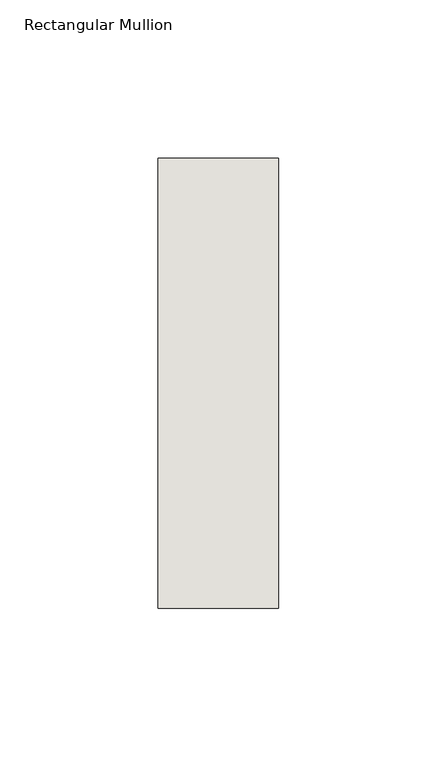
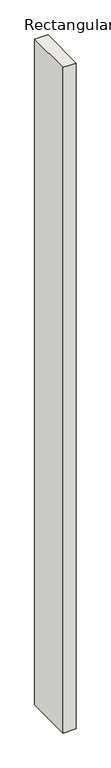
"""IFC4 building model written with IfcOpenShell, lengths in millimetres: wall geometry, Rectangular Mullion : NLRS_21_CWM_hsb-regel 38x142_gen_rsf."""

from ifc_helpers import new_model, si_unit, frame, origin, place, context, project, spatial, polyline, outline, extrude, source, transform, mapped, element, save


def rectangular_mullion_b4280be7(model_context):
    return source(origin(), model_context, "Body", "SweptSolid", [
        extrude(outline(polyline([(-38.0, -71.0), (-38.0, 71.0), (0.0, 71.0), (0.0, -71.0), (-38.0, -71.0)])), frame((0.0, 0.0, -2038.0), z_axis=(0.0, 0.0, 1.0), x_axis=(1.0, 0.0, 0.0)), (0.0, 0.0, 1.0), 2038.0),
    ])


if __name__ == "__main__":
    model = new_model("IFC4")
    model_context = context("Model", 3, world=origin())
    ifc_project = project(units=[si_unit("LENGTHUNIT", "METRE", prefix="MILLI")], contexts=[model_context])
    site = spatial("IfcSite", under=ifc_project)
    building = spatial("IfcBuilding", under=site)
    placement = place(None, origin())
    rectangular_mullion_shape = rectangular_mullion_b4280be7(model_context)
    element("IfcWall", 1, ObjectType="Rectangular Mullion : NLRS_21_CWM_hsb-regel 38x142_gen_rsf", at=placement, inside=building, context=model_context, shape_type="MappedRepresentation", body=[
        mapped(rectangular_mullion_shape, transform((0.0, 0.0, 0.0), x_axis=(1.0, 0.0, 0.0), y_axis=(0.0, 1.0, 0.0), z_axis=(0.0, 0.0, 1.0))),
    ])
    save(model, "model.ifc")

# Revit data of these elements
# Type "Rectangular Mullion : NLRS_21_CWM_hsb-regel 38x142_gen_rsf"
#   Type IfcGUID = "07M7mRoiH1CR8m_RSKIwpF"
#   Assembly Code = "21.10"
#   IfcExportAs = "IfcWall"
#   built-in parameter 1007322 = 0.465879 (stored number, unit not read)
#   built-in parameter 1007321 = 0.062336 (stored number, unit not read)
#   built-in parameter 1007320 = 0.062336 (stored number, unit not read)
# Element 1 (IfcWall, "Rectangular Mullion : NLRS_21_CWM_hsb-regel 38x142_gen_rsf")
#   Materials on its faces: "NLRS_i2_hout naaldhout vuren_gen_rsf"
# Materials
#   "NLRS_i2_hout naaldhout vuren_gen_rsf": class "I - Hout", colour RGB 234 199 147, transparency 0, Keynote = "i2", Manufacturer = "Revit Standards Foundation", URL = "www.revitstandards.org", Description = "hout vuren", Cost = 0
